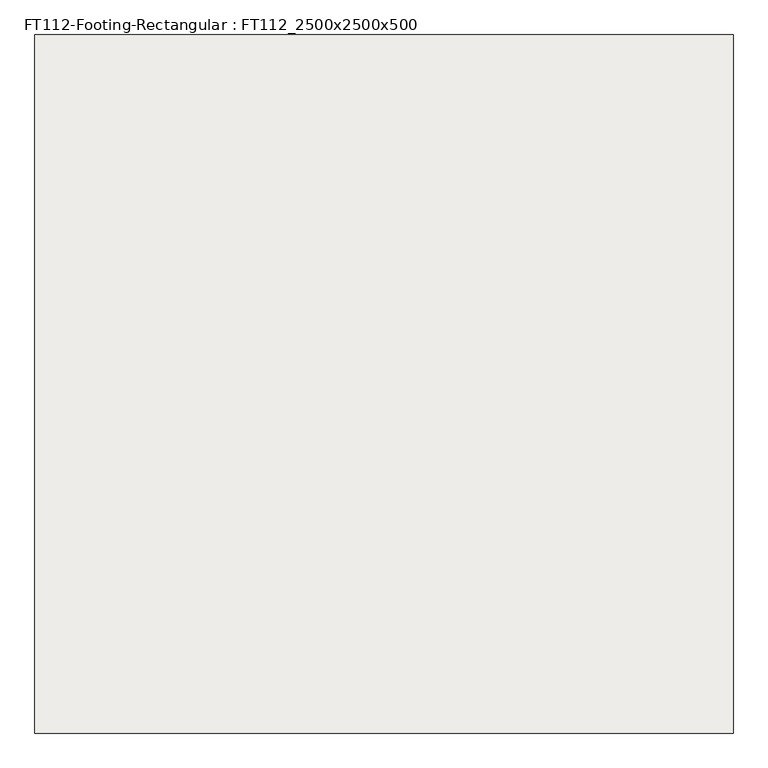
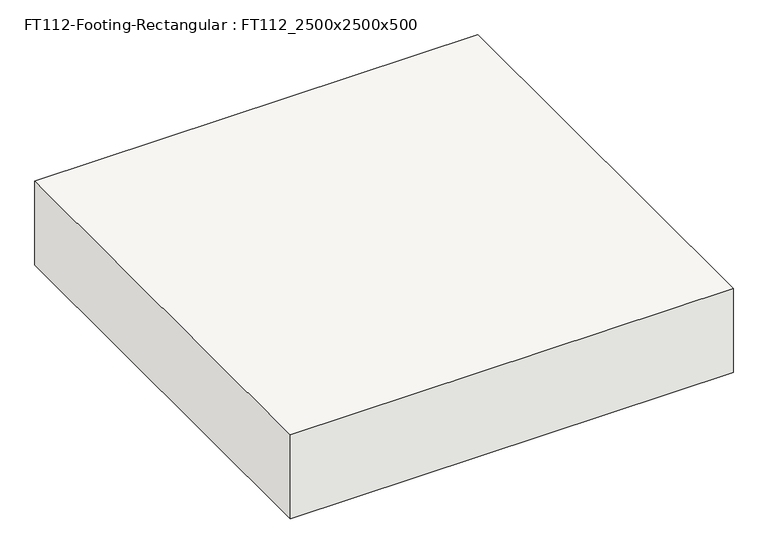
"""IFC4 building model written with IfcOpenShell, lengths in millimetres: slab geometry, FT112-Footing-Rectangular : FT112_2500x2500x500."""

from ifc_helpers import new_model, si_unit, frame, origin, place, context, project, spatial, polyline, outline, extrude, source, transform, mapped, element, save


def ft112_footing_rectangular_ft112_2500x2500x500_513089b3(model_context):
    return source(origin(), model_context, "Body", "SweptSolid", [
        extrude(outline(polyline([(1250.0, 1250.0), (1250.0, -1250.0), (-1250.0, -1250.0), (-1250.0, 1250.0), (1250.0, 1250.0)])), frame((0.0, 0.0, -500.0), z_axis=(0.0, 0.0, 1.0), x_axis=(1.0, 0.0, 0.0)), (0.0, 0.0, 1.0), 500.0),
    ])


if __name__ == "__main__":
    model = new_model("IFC4")
    model_context = context("Model", 3, world=origin())
    ifc_project = project(units=[si_unit("LENGTHUNIT", "METRE", prefix="MILLI")], contexts=[model_context])
    site = spatial("IfcSite", under=ifc_project)
    building = spatial("IfcBuilding", under=site)
    placement = place(None, origin())
    ft112_footing_rectangular_ft112_2500x2500x500_shape = ft112_footing_rectangular_ft112_2500x2500x500_513089b3(model_context)
    element("IfcSlab", 1, ObjectType="FT112-Footing-Rectangular : FT112_2500x2500x500", at=placement, inside=building, context=model_context, shape_type="MappedRepresentation", body=[
        mapped(ft112_footing_rectangular_ft112_2500x2500x500_shape, transform((0.0, 0.0, 0.0), x_axis=(1.0, 0.0, 0.0), y_axis=(0.0, 1.0, 0.0), z_axis=(0.0, 0.0, 1.0))),
    ])
    save(model, "model.ifc")

# Revit data of these elements
# Type "FT112-Footing-Rectangular : FT112_2500x2500x500"
#   Description = "UG Shallow Foundation"
#   Width = 2500 mm
#   Length = 2500 mm
#   Foundation Thickness = 500 mm
#   hec_material3 [instance default] = none
#   hec_material2 [instance default] = A03AE056-00001_Bitumen/Bituminous/Asphalt Coating
#   hec_material1 [instance default] = A03AC035-00001_Form Work (3 times in use)_Flat
#   Structural Material [instance default] = A03AC032-00007_Structural Concrete_Type1_25MPa-30Mpa
#   Assembly Code = ""
# Element 1 (IfcSlab, "FT112-Footing-Rectangular : FT112_2500x2500x500")
#   Structural Material = 콘크리트 - 현장타설 콘크리트
#   Materials on its faces: "콘크리트 - 현장타설 콘크리트"
# Materials
#   "A03AE056-00001_Bitumen/Bituminous/Asphalt Coating": class "Generic", colour RGB 17 17 17, transparency 0, Description = "Damp-proofing", W00) Work Master Code = "A03AE056-00001", W01) Work Master_Lv1 = "Concrete Work", W02) Work Master_Lv2 = "Concrete Protective Coating (U/G)", W03) Work Master_Spec.1 = "Bitumen/Bituminous/Asphalt Coating", Cost = 0
#   "A03AC035-00001_Form Work (3 times in use)_Flat": class "Wood", colour RGB 149 120 74, transparency 0, Description = "Plywood", W00) Work Master Code = "A03AC035-00001", W01) Work Master_Lv1 = "Concrete Work", W02) Work Master_Lv2 = "Substructure Work", W03) Work Master_Spec.1 = "Form Work (3 times in use)", W04) Work Master_Spec.2 = "Flat Form", W05) Work Master_Spec.3 = "Dressed Lumber, Plywood or Steel Form(Wood Planks are not Allowed) incl. Chamfer", Cost = 0
#   "A03AC032-00007_Structural Concrete_Type1_25MPa-30Mpa": class "Concrete", colour RGB 176 176 176, transparency 0, Keynote = "09910.A1", Description = "Reinf. Conc.", W00) Work Master Code = "A03AC032-00007", W01) Work Master_Lv1 = "Concrete Work", W02) Work Master_Lv2 = "Substructure Work", W03) Work Master_Spec.1 = "Structural Concrete", W04) Work Master_Spec.2 = "Cement Type-1", W05) Work Master_Spec.3 = "25MPa < F'c (Cylinder Strength) ≤ 30MPa", Cost = 0
#   "콘크리트 - 현장타설 콘크리트": class "콘크리트", colour RGB 192 192 192, transparency 0, Cost = 0
